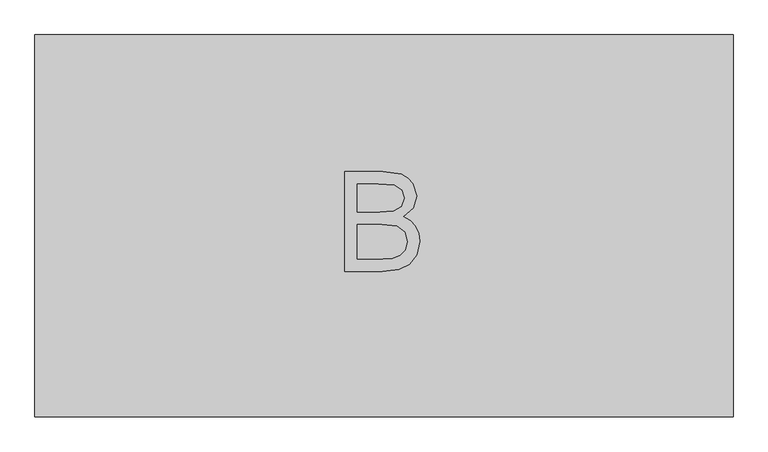
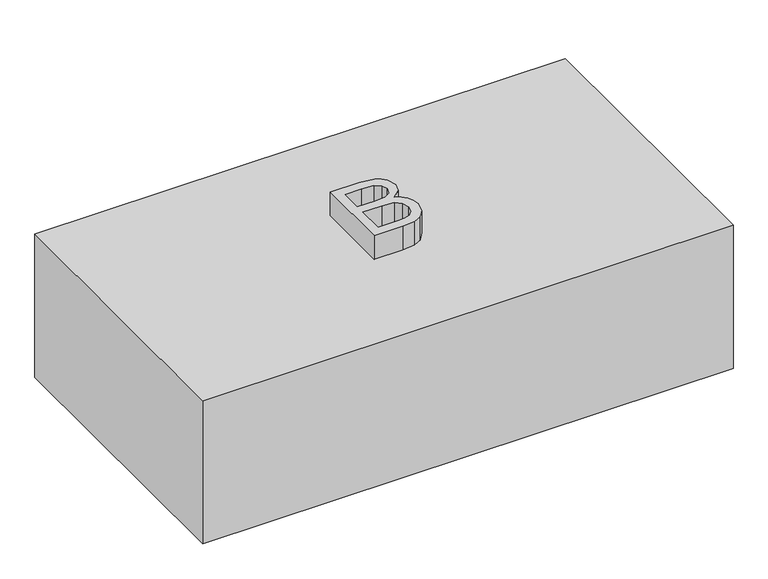
"""IFC4 building model written with IfcOpenShell, lengths in millimetres: proxy geometry, The Messy Family B : The Messy Family B."""

from ifc_helpers import new_model, si_unit, frame, origin, origin_with_axes, place, context, project, spatial, polyline, outline, extrude, source, transform, mapped, element, save


def generic_models_ac3e04e5(model_context):
    return source(origin(), model_context, "Body", "SweptSolid", [
        extrude(outline(polyline([(541.9415527, 284.565081), (541.9415527, -299.634919), (-524.8584473, -299.634919), (-524.8584473, 284.565081), (541.9415527, 284.565081)])), origin_with_axes(), (0.0, 0.0, 1.0), 304.8),
        extrude(outline(polyline([(-51.7602961, -77.2556777), (-51.7602961, 75.839739), (6.6596591, 75.839739), (35.2716077, 71.3358333), (44.8867922, 65.6218534), (52.1659261, 57.4877249), (58.2770347, 37.9022761), (53.1377232, 20.0174722), (37.6076583, 6.4683783), (48.4516055, 0.8057915), (56.4642593, -7.8095634), (61.4120147, -18.8076899), (63.0612664, -31.6185918), (58.5573607, -52.1945261), (47.4003827, -66.8462359), (30.7490136, -74.6206125), (6.2111373, -77.2556777), (-51.7602961, -77.2556777)]), holes=[polyline([(-32.623369, 13.644726), (2.323949, 13.644726), (22.7316877, 15.2893056), (35.00997, 22.3722113), (39.1401076, 34.8373776), (35.2902961, 47.3212324), (24.2641369, 54.7031525), (-0.3298045, 56.7028119), (-32.623369, 56.7028119), (-32.623369, 13.644726)]), polyline([(-32.623369, -58.1187506), (6.6222823, -58.1187506), (20.8254703, -57.3712144), (32.842115, -53.2037), (40.8033757, -44.7004755), (43.9243394, -31.8054758), (40.2614119, -16.9295052), (28.3942745, -8.0525126), (4.7534417, -5.4922011), (-32.623369, -5.4922011), (-32.623369, -58.1187506)])]), frame((0.0, 0.0, 304.8), z_axis=(0.0, 0.0, 1.0), x_axis=(1.0, 0.0, 0.0)), (0.0, 0.0, 1.0), 50.8),
    ])


if __name__ == "__main__":
    model = new_model("IFC4")
    model_context = context("Model", 3, world=origin())
    ifc_project = project(units=[si_unit("LENGTHUNIT", "METRE", prefix="MILLI")], contexts=[model_context])
    site = spatial("IfcSite", under=ifc_project)
    building = spatial("IfcBuilding", under=site)
    placement = place(None, origin())
    generic_models_shape = generic_models_ac3e04e5(model_context)
    element("IfcBuildingElementProxy", 1, Name="The Messy Family B : The Messy Family B", ObjectType="The Messy Family B : The Messy Family B", at=placement, inside=building, context=model_context, shape_type="MappedRepresentation", body=[
        mapped(generic_models_shape, transform((0.0, 0.0, 0.0), x_axis=(1.0, 0.0, 0.0), y_axis=(0.0, 1.0, 0.0), z_axis=(0.0, 0.0, 1.0))),
    ])
    save(model, "model.ifc")

# Revit data of these elements
# Type "The Messy Family B : The Messy Family B"
#   TBC-Parameter 2 = ""
#   TBC-Parameter 1 = ""
#   Other Company Parameter 2 = ""
#   Other Company Parameter 1 = ""
#   TBC-Parameter 3 = 2' - 0"
#   Other Company Parameter 3 = 1' - 0"
#   Default Elevation = 0
